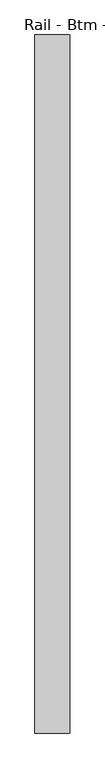
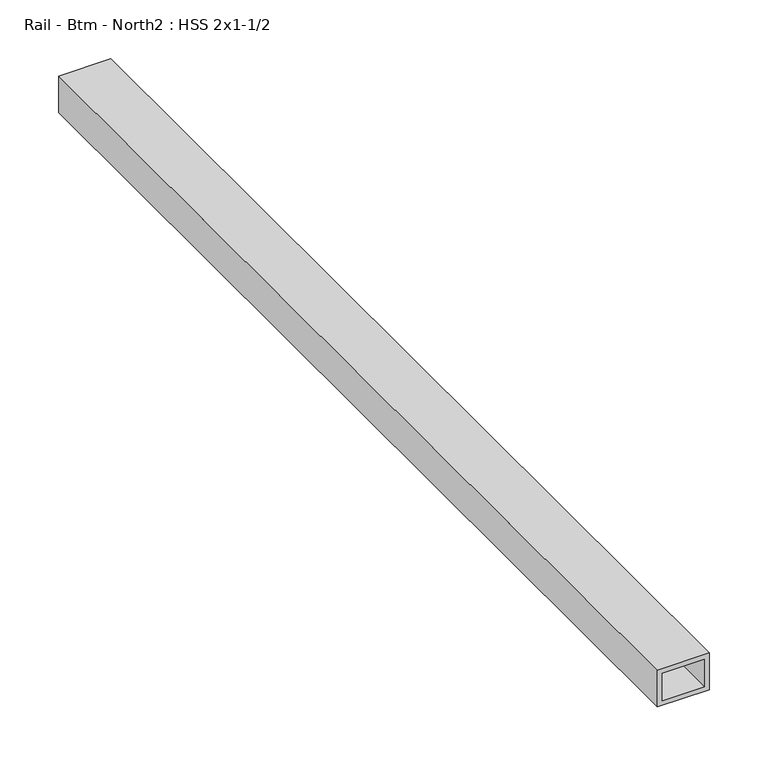
"""IFC4 building model written with IfcOpenShell, lengths in millimetres: proxy geometry, Rail - Btm - North2 : HSS 2x1-1/2."""

from ifc_helpers import new_model, si_unit, frame, origin, place, context, project, spatial, polyline, outline, extrude, source, transform, mapped, element, save


def rail_btm_north2_hss_2x1_1_2_b7e517c1(model_context):
    return source(origin(), model_context, "Body", "SweptSolid", [
        extrude(outline(polyline([(50.8, 587416.6934739), (88.9, 587416.6934739), (88.9, 587365.8934739), (50.8, 587365.8934739), (50.8, 587416.6934739)]), holes=[polyline([(84.1375, 587411.9309739), (55.5625, 587411.9309739), (55.5625, 587370.6559739), (84.1375, 587370.6559739), (84.1375, 587411.9309739)])]), frame((0.0, -532839.3663841, 0.0), z_axis=(0.0, 1.0, 0.0), x_axis=(0.0, 0.0, 1.0)), (0.0, 0.0, 1.0), 1016.0),
    ])


if __name__ == "__main__":
    model = new_model("IFC4")
    model_context = context("Model", 3, world=origin())
    ifc_project = project(units=[si_unit("LENGTHUNIT", "METRE", prefix="MILLI")], contexts=[model_context])
    site = spatial("IfcSite", under=ifc_project)
    building = spatial("IfcBuilding", under=site)
    placement = place(None, origin())
    rail_btm_north2_hss_2x1_1_2_shape = rail_btm_north2_hss_2x1_1_2_b7e517c1(model_context)
    element("IfcBuildingElementProxy", 1, Name="Rail - Btm - North2 : HSS 2x1-1/2", ObjectType="Rail - Btm - North2 : HSS 2x1-1/2", at=placement, inside=building, context=model_context, shape_type="MappedRepresentation", body=[
        mapped(rail_btm_north2_hss_2x1_1_2_shape, transform((0.0, 0.0, 0.0), x_axis=(1.0, 0.0, 0.0), y_axis=(0.0, 1.0, 0.0), z_axis=(0.0, 0.0, 1.0))),
    ])
    save(model, "model.ifc")

# Revit data of these elements
# Element 1 (IfcBuildingElementProxy, "Rail - Btm - North2 : HSS 2x1-1/2")
#   Materials on its faces: "1-1/2\"X2\" GALV. STL HSS TUBING"
# Materials
#   "1-1/2\"X2\" GALV. STL HSS TUBING": class "Generic", colour RGB 211 211 207, transparency 0, Cost = 0
